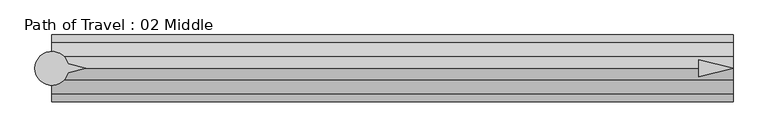
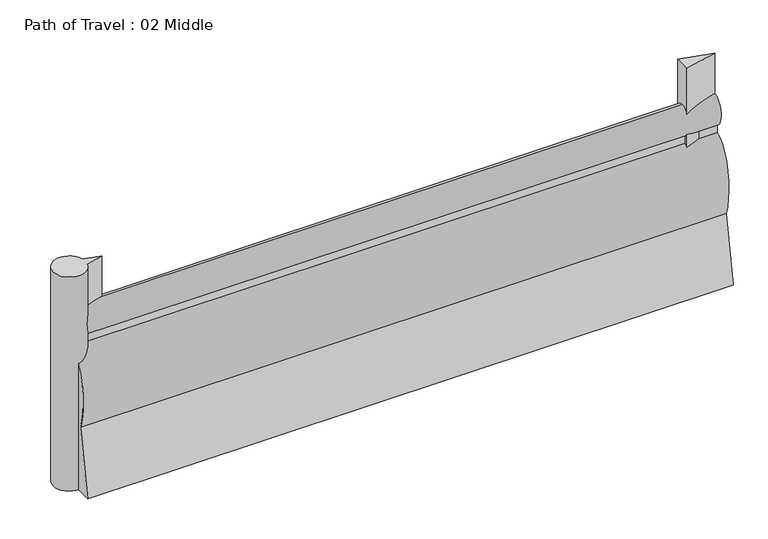
"""IFC4 building model written with IfcOpenShell, lengths in millimetres: proxy geometry, Path of Travel : 02 Middle."""

from ifc_helpers import new_model, si_unit, point, frame, frame_2d, origin, origin_with_axes, place, context, project, spatial, polyline, circle_curve, ellipse_curve, trimmed, segment, composite_curve, outline, extrude, source, transform, mapped, element, save
from ifc_brep_helpers import plane_surface, extruded_surface, advanced_brep


def path_of_travel_02_middle_7e98c3bf(model_context):
    return source(origin(), model_context, "Body", "SolidModel", [
        advanced_brep(
        [(227.5554837, 0.0, 1727.2), (227.5554837, 42.9018657, 1436.6534209), (227.5554837, 42.9018657, 1363.4763406), (227.5554837, 184.1186263, 643.4144547), (227.5554837, 297.5699544, 0.0), (227.5554837, 145.6574193, 0.0), (227.5554837, 0.0, 584.2), (227.5554837, -145.6574193, 0.0), (227.5554837, -297.5699544, 0.0), (227.5554837, -184.1186263, 643.4144547), (227.5554837, -42.9018657, 1363.4763406), (227.5554837, -42.9018657, 1436.6534209), (6298.8639119, 0.0, 1727.2), (6298.8639119, -42.9018657, 1436.6534209), (6298.8639119, -42.9018657, 1363.4763406), (6298.8639119, -184.1186263, 643.4144547), (6298.8639119, -297.5699544, 0.0), (6298.8639119, -145.6574193, 0.0), (6298.8639119, 0.0, 584.2), (6298.8639119, 145.6574193, 0.0), (6298.8639119, 297.5699544, 0.0), (6298.8639119, 184.1186263, 643.4144547), (6298.8639119, 42.9018657, 1363.4763406), (6298.8639119, 42.9018657, 1436.6534209)],
        [
            (0, 1, ellipse_curve(frame((227.5554837, 0.0, 1574.8), z_axis=(-1.0, 0.0, 0.0), x_axis=(0.0, 0.0, 1.0)), 152.4, 101.6)),
            (1, 2),
            (2, 3, ellipse_curve(frame((227.5554837, 0.0, 914.4), z_axis=(-1.0, 0.0, 0.0), x_axis=(0.0, 0.0, -1.0)), 457.2, 228.6)),
            (3, 4),
            (4, 5),
            (5, 6),
            (6, 7),
            (7, 8),
            (8, 9),
            (9, 10, ellipse_curve(frame((227.5554837, 0.0, 914.4), z_axis=(-1.0, 0.0, 0.0), x_axis=(0.0, 0.0, -1.0)), 457.2, 228.6)),
            (10, 11),
            (11, 0, ellipse_curve(frame((227.5554837, 0.0, 1574.8), z_axis=(-1.0, 0.0, 0.0), x_axis=(0.0, 0.0, 1.0)), 152.4, 101.6)),
            (12, 13, ellipse_curve(frame((6298.8639119, 0.0, 1574.8), z_axis=(1.0, 0.0, 0.0), x_axis=(0.0, 0.0, 1.0)), 152.4, 101.6)),
            (13, 14),
            (14, 15, ellipse_curve(frame((6298.8639119, 0.0, 914.4), z_axis=(1.0, 0.0, 0.0), x_axis=(0.0, 0.0, -1.0)), 457.2, 228.6)),
            (15, 16),
            (16, 17),
            (17, 18),
            (18, 19),
            (19, 20),
            (20, 21),
            (21, 22, ellipse_curve(frame((6298.8639119, 0.0, 914.4), z_axis=(1.0, 0.0, 0.0), x_axis=(0.0, 0.0, -1.0)), 457.2, 228.6)),
            (22, 23),
            (23, 12, ellipse_curve(frame((6298.8639119, 0.0, 1574.8), z_axis=(1.0, 0.0, 0.0), x_axis=(0.0, 0.0, 1.0)), 152.4, 101.6)),
            (0, 12),
            (23, 1),
            (22, 2),
            (21, 3),
            (20, 4),
            (19, 5),
            (18, 6),
            (17, 7),
            (16, 8),
            (15, 9),
            (14, 10),
            (13, 11),
        ],
        [
            plane_surface(frame((227.5554837, 0.0, 0.0), z_axis=(-1.0, 0.0, 0.0), x_axis=(0.0, 0.0, 1.0))),
            plane_surface(frame((6298.8639119, 0.0, 0.0), z_axis=(1.0, 0.0, 0.0), x_axis=(0.0, 0.0, 1.0))),
            extruded_surface(trimmed(ellipse_curve(frame((6298.8639119, 0.0, 1574.8), z_axis=(-1.0, 0.0, 0.0), x_axis=(0.0, 0.0, 1.0)), 152.4, 101.6), [point((6298.8639119, 0.0, 1727.2))], [point((6298.8639119, 42.9018657, 1436.6534209))], True, "CARTESIAN"), (-6071.3084282, 0.0, 0.0), 6071.3084282),
            plane_surface(frame((227.5554837, 42.9018657, 1436.6534209), z_axis=(0.0, 1.0, 0.0), x_axis=(1.0, 0.0, 0.0))),
            extruded_surface(trimmed(ellipse_curve(frame((6298.8639119, 0.0, 914.4), z_axis=(-1.0, 0.0, 0.0), x_axis=(0.0, 0.0, -1.0)), 457.2, 228.6), [point((6298.8639119, 42.9018657, 1363.4763406))], [point((6298.8639119, 184.1186263, 643.4144547))], True, "CARTESIAN"), (-6071.3084282, 0.0, 0.0), 6071.3084282),
            plane_surface(frame((227.5554837, 184.1186263, 643.4144547), z_axis=(0.0, 0.9848077530122078, 0.1736481776669322), x_axis=(1.0, 0.0, 0.0))),
            plane_surface(frame((227.5554837, 297.5699544, 0.0), z_axis=(0.0, 0.0, -1.0), x_axis=(1.0, 0.0, 0.0))),
            plane_surface(frame((227.5554837, 145.6574193, 0.0), z_axis=(0.0, -0.9702957262760199, -0.2419218955995739), x_axis=(1.0, 0.0, 0.0))),
            plane_surface(frame((227.5554837, 0.0, 584.2), z_axis=(0.0, 0.9702957262759961, -0.24192189559966923), x_axis=(1.0, 0.0, 0.0))),
            plane_surface(frame((227.5554837, -145.6574193, 0.0), z_axis=(0.0, 0.0, -1.0), x_axis=(1.0, 0.0, 0.0))),
            plane_surface(frame((227.5554837, -297.5699544, 0.0), z_axis=(0.0, -0.984807753012208, 0.17364817766693066), x_axis=(1.0, 0.0, 0.0))),
            extruded_surface(trimmed(ellipse_curve(frame((6298.8639119, 0.0, 914.4), z_axis=(-1.0, 0.0, 0.0), x_axis=(0.0, 0.0, -1.0)), 457.2, 228.6), [point((6298.8639119, -184.1186263, 643.4144547))], [point((6298.8639119, -42.9018657, 1363.4763406))], True, "CARTESIAN"), (-6071.3084282, 0.0, 0.0), 6071.3084282),
            plane_surface(frame((227.5554837, -42.9018657, 1363.4763406), z_axis=(0.0, -1.0, 0.0), x_axis=(1.0, 0.0, 0.0))),
            extruded_surface(trimmed(ellipse_curve(frame((6298.8639119, 0.0, 1574.8), z_axis=(-1.0, 0.0, 0.0), x_axis=(0.0, 0.0, 1.0)), 152.4, 101.6), [point((6298.8639119, -42.9018657, 1436.6534209))], [point((6298.8639119, 0.0, 1727.2))], True, "CARTESIAN"), (-6071.3084282, 0.0, 0.0), 6071.3084282),
        ],
        [
            (0, [[1, 2, 3, 4, 5, 6, 7, 8, 9, 10, 11, 12]]),
            (1, [[13, 14, 15, 16, 17, 18, 19, 20, 21, 22, 23, 24]]),
            (2, [[-1, 25, -24, 26]]),
            (3, [[-2, -26, -23, 27]]),
            (4, [[-3, -27, -22, 28]]),
            (5, [[-4, -28, -21, 29]]),
            (6, [[-5, -29, -20, 30]]),
            (7, [[-6, -30, -19, 31]]),
            (8, [[-7, -31, -18, 32]]),
            (9, [[-8, -32, -17, 33]]),
            (10, [[-9, -33, -16, 34]]),
            (11, [[-10, -34, -15, 35]]),
            (12, [[-11, -35, -14, 36]]),
            (13, [[-12, -36, -13, -25]]),
        ],
    ),
        extrude(outline(polyline([(5992.8587653, 76.2006338), (6298.8639119, 0.0), (5992.8587653, -76.2006338), (5992.8587653, 76.2006338)])), origin_with_axes(), (0.0, 0.0, 1.0), 2129.5973753),
        extrude(outline(composite_curve([segment(polyline([(372.7837828, 39.4440225), (531.182385, 0.0), (372.7837828, -39.4440225)]), True, "CONTINUOUS"), segment(trimmed(circle_curve(frame_2d((227.2200886, 0.0)), 150.8131956), [point((372.7837828, -39.4440225))], [point((372.7837828, 39.4440225))], False, "CARTESIAN"), True, "CONTINUOUS")], self_intersect=False)), origin_with_axes(), (0.0, 0.0, 1.0), 2129.5973753),
    ])


if __name__ == "__main__":
    model = new_model("IFC4")
    model_context = context("Model", 3, world=origin())
    ifc_project = project(units=[si_unit("LENGTHUNIT", "METRE", prefix="MILLI")], contexts=[model_context])
    site = spatial("IfcSite", under=ifc_project)
    building = spatial("IfcBuilding", under=site)
    placement = place(None, origin())
    path_of_travel_02_middle_shape = path_of_travel_02_middle_7e98c3bf(model_context)
    element("IfcBuildingElementProxy", 1, Name="Path of Travel : 02 Middle", ObjectType="Path of Travel : 02 Middle", at=placement, inside=building, context=model_context, shape_type="MappedRepresentation", body=[
        mapped(path_of_travel_02_middle_shape, transform((0.0, 0.0, 0.0), x_axis=(1.0, 0.0, 0.0), y_axis=(0.0, 1.0, 0.0), z_axis=(0.0, 0.0, 1.0))),
    ])
    save(model, "model.ifc")

# Revit data of these elements
# Type "Path of Travel : 02 Middle"
#   Path of Egress [instance default] = 4' - 0"
#   built-in parameter 1001306 [instance default] = 4 (stored number, unit not read)
#   Dot at Start = no
#   Arrow in Middle = yes
#   Arrow at End = no
#   Egress Path = none
# Element 1 (IfcBuildingElementProxy, "Path of Travel : 02 Middle")
#   Path of Egress = 19' - 11.02789"
#   built-in parameter 1001306 = 19.919 (stored number, unit not read)
